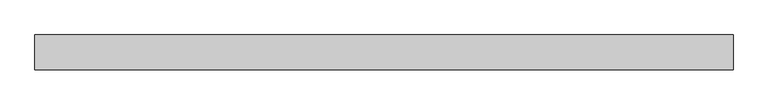
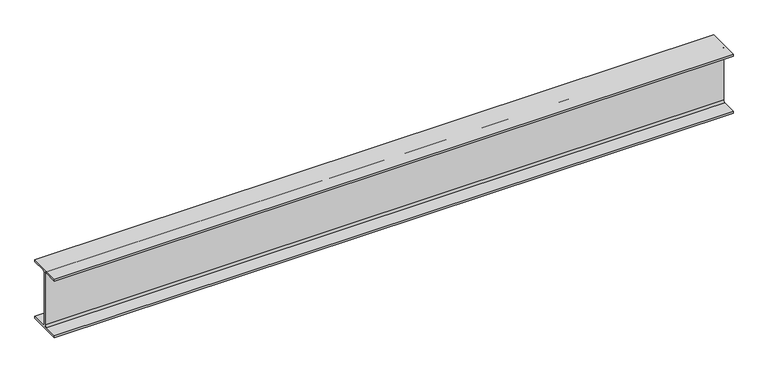
"""IFC4 building model written with IfcOpenShell, lengths in millimetres: beam geometry, Old_Steel Beam_H-KSD3502 : H_SB_ASB_H-200×200x8x12."""

from ifc_helpers import new_model, si_unit, point, frame, frame_2d, origin, place, context, project, spatial, polyline, circle_curve, trimmed, segment, composite_curve, outline, extrude, source, transform, mapped, element, save


def beam_5e19d841(model_context):
    return source(origin(), model_context, "Body", "SweptSolid", [
        extrude(outline(composite_curve([segment(polyline([(82.5, -141.5), (82.5, -151.7), (-82.5, -151.7), (-82.5, -141.5), (-11.9, -141.5)]), True, "CONTINUOUS"), segment(trimmed(circle_curve(frame_2d((-11.9, -132.6)), 8.9), [point((-11.9, -141.5))], [point((-3.0, -132.6))], True, "CARTESIAN"), True, "CONTINUOUS"), segment(polyline([(-3.0, -132.6), (-3.0, 132.6)]), True, "CONTINUOUS"), segment(trimmed(circle_curve(frame_2d((-11.9, 132.6)), 8.9), [point((-3.0, 132.6))], [point((-11.9, 141.5))], True, "CARTESIAN"), True, "CONTINUOUS"), segment(polyline([(-11.9, 141.5), (-82.5, 141.5), (-82.5, 151.7), (82.5, 151.7), (82.5, 141.5), (11.9, 141.5)]), True, "CONTINUOUS"), segment(trimmed(circle_curve(frame_2d((11.9, 132.6)), 8.9), [point((11.9, 141.5))], [point((3.0, 132.6))], True, "CARTESIAN"), True, "CONTINUOUS"), segment(polyline([(3.0, 132.6), (3.0, -132.6)]), True, "CONTINUOUS"), segment(trimmed(circle_curve(frame_2d((11.9, -132.6)), 8.9), [point((3.0, -132.6))], [point((11.9, -141.5))], True, "CARTESIAN"), True, "CONTINUOUS"), segment(polyline([(11.9, -141.5), (82.5, -141.5)]), True, "CONTINUOUS")], self_intersect=False)), frame((-1721.7329802, 0.0, 0.0), z_axis=(1.0, 0.0, 0.0), x_axis=(0.0, 1.0, 0.0)), (0.0, 0.0, 1.0), 3316.0486402),
    ])


if __name__ == "__main__":
    model = new_model("IFC4")
    model_context = context("Model", 3, world=origin())
    ifc_project = project(units=[si_unit("LENGTHUNIT", "METRE", prefix="MILLI")], contexts=[model_context])
    site = spatial("IfcSite", under=ifc_project)
    building = spatial("IfcBuilding", under=site)
    placement = place(None, origin())
    beam_shape = beam_5e19d841(model_context)
    element("IfcBeam", 1, ObjectType="Old_Steel Beam_H-KSD3502 : H_SB_ASB_H-200×200x8x12", at=placement, inside=building, context=model_context, shape_type="MappedRepresentation", body=[
        mapped(beam_shape, transform((0.0, 0.0, 0.0), x_axis=(1.0, 0.0, 0.0), y_axis=(0.0, 1.0, 0.0), z_axis=(0.0, 0.0, 1.0))),
    ])
    save(model, "model.ifc")

# Revit data of these elements
# Type "Old_Steel Beam_H-KSD3502 : H_SB_ASB_H-200×200x8x12"
#   Width = 20.0 cm
#   Web Thickness = 0.8 cm
#   Web Fillet = 1.3 cm
#   Warping Constant = 141376.0 cm⁶
#   Torsional Moment of Inertia = 26.2485 cm⁴
#   Torsional Modulus = 1.0 cm³
#   Section Area = 63.53 cm²
#   Plastic Modulus weak axis = 244.0 cm³
#   Plastic Modulus strong axis = 525.0 cm³
#   Perimeter = 1.16 m²/m
#   Nominal Weight = 49.90 kgf/m
#   Moment of Inertia weak axis = 1600.00 cm⁴
#   Moment of Inertia strong axis = 4720.00 cm⁴
#   Height = 20.0 cm
#   Flange Thickness = 1.2 cm
#   Elastic Modulus weak axis = 160.0 cm³
#   Elastic Modulus strong axis = 472.0 cm³
#   Centroid Vertical = 10.0 cm
#   Centroid Horizontal = 10.0 cm
#   Length [instance default] = 1.5240 m
#   Structural Material [instance default] = Steel, 45-345
#   Assembly Code = ""
# Element 1 (IfcBeam, "Old_Steel Beam_H-KSD3502 : H_SB_ASB_H-200×200x8x12")
#   Structural Material = none
# Materials
#   "Steel, 45-345": class "Metal", colour RGB 189 187 185, transparency 0, Description = "Steel 345 MPa", Cost = 0
